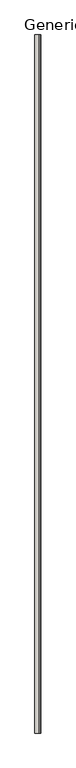
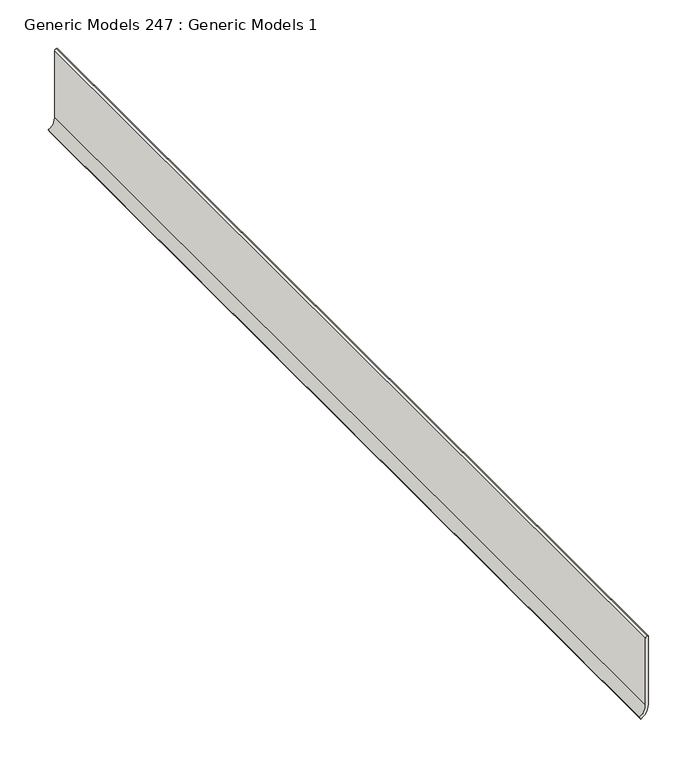
"""IFC4 building model written with IfcOpenShell, lengths in millimetres: wall geometry, Generic Models 247 : Generic Models 1."""

from ifc_helpers import new_model, si_unit, point, frame, frame_2d, origin, place, context, project, spatial, polyline, circle_curve, trimmed, segment, composite_curve, outline, extrude, source, transform, mapped, element, save


def generic_models_247_generic_models_1_1e199e3a(model_context):
    return source(origin(), model_context, "Body", "SweptSolid", [
        extrude(outline(composite_curve([segment(polyline([(3149.6, 49679.225), (3149.6, 49678.1368018)]), True, "CONTINUOUS"), segment(trimmed(circle_curve(frame_2d((3147.5131982, 49678.1368018)), 2.0868018), [point((3149.6, 49678.1368018))], [point((3147.5131982, 49676.05))], False, "CARTESIAN"), True, "CONTINUOUS"), segment(polyline([(3147.5131982, 49676.05), (3063.4496307, 49676.05)]), True, "CONTINUOUS"), segment(trimmed(circle_curve(frame_2d((3063.4496307, 49661.3853032)), 14.6646968), [point((3063.4496307, 49676.05))], [point((3050.7496307, 49668.7176516))], True, "CARTESIAN"), True, "CONTINUOUS"), segment(polyline([(3050.7496307, 49668.7176516), (3048.0, 49670.3051516)]), True, "CONTINUOUS"), segment(trimmed(circle_curve(frame_2d((3063.4496307, 49661.3853032)), 17.8396968), [point((3048.0, 49670.3051516))], [point((3063.4496307, 49679.225))], False, "CARTESIAN"), True, "CONTINUOUS"), segment(polyline([(3063.4496307, 49679.225), (3149.6, 49679.225)]), True, "CONTINUOUS")], self_intersect=False)), frame((0.0, 0.0, 0.0), z_axis=(0.0, 1.0, 0.0), x_axis=(0.0, 0.0, 1.0)), (0.0, 0.0, 1.0), 1219.2),
    ])


if __name__ == "__main__":
    model = new_model("IFC4")
    model_context = context("Model", 3, world=origin())
    ifc_project = project(units=[si_unit("LENGTHUNIT", "METRE", prefix="MILLI")], contexts=[model_context])
    site = spatial("IfcSite", under=ifc_project)
    building = spatial("IfcBuilding", under=site)
    placement = place(None, origin())
    generic_models_247_generic_models_1_shape = generic_models_247_generic_models_1_1e199e3a(model_context)
    element("IfcWall", 1, ObjectType="Generic Models 247 : Generic Models 1", at=placement, inside=building, context=model_context, shape_type="MappedRepresentation", body=[
        mapped(generic_models_247_generic_models_1_shape, transform((0.0, 0.0, 0.0), x_axis=(1.0, 0.0, 0.0), y_axis=(0.0, 1.0, 0.0), z_axis=(0.0, 0.0, 1.0))),
    ])
    save(model, "model.ifc")

# Revit data of these elements
# Element 1 (IfcWall, "Generic Models 247 : Generic Models 1")
#   Materials on its faces: "MATCH EXISTING BASE"
# Materials
#   "MATCH EXISTING BASE": class "Generic", colour RGB 120 120 120, transparency 0, Cost = 0
